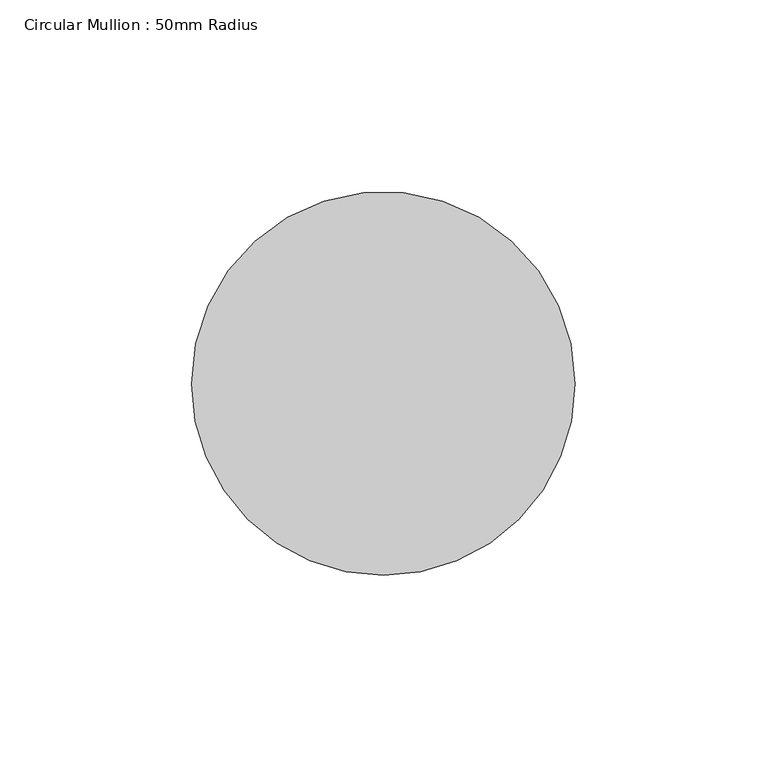
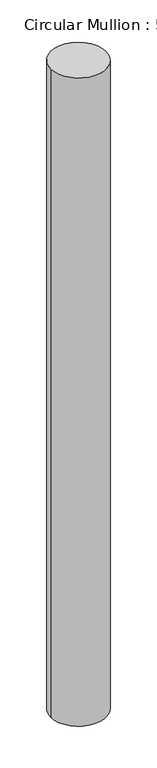
"""IFC4 building model written with IfcOpenShell, lengths in millimetres: member geometry, Circular Mullion : 50mm Radius."""

from ifc_helpers import new_model, si_unit, frame, origin, place, context, project, spatial, ellipse_curve, source, transform, mapped, element, save
from ifc_brep_helpers import plane_surface, cylinder_surface, advanced_brep


def circular_mullion_50mm_radius_11ac74c6(model_context):
    return source(origin(), model_context, "Body", "AdvancedBrep", [
        advanced_brep(
        [(-100.0, 0.0, 0.6910365), (0.0, 0.0, 0.0), (0.0, 0.0, -1242.7098451), (-100.0, 0.0, -1243.4311044)],
        [
            (0, 1, ellipse_curve(frame((-50.0, 0.0, 0.3455183), z_axis=(-0.006909628578011499, -0.012865343381346107, -0.999893364300711), x_axis=(-0.47310077416802043, -0.88088727851764, 0.014603425194297921)), 50.0053324, 50.0)),
            (1, 2),
            (2, 3, ellipse_curve(frame((-50.0, 0.0, -1243.0704748), z_axis=(-0.007211755555192615, -0.013427886977189473, 0.9998838344693548), x_axis=(0.4730962651165488, 0.8808788829151897, 0.015241967289685193)), 50.005809, 50.0)),
            (3, 0),
            (1, 0, ellipse_curve(frame((-50.0, 0.0, 0.3455183), z_axis=(-0.006909628578011499, -0.012865343381346107, -0.999893364300711), x_axis=(-0.47310077416802043, -0.88088727851764, 0.014603425194297921)), 50.0053324, 50.0)),
            (3, 2, ellipse_curve(frame((-50.0, 0.0, -1243.0704748), z_axis=(-0.007211755555192615, -0.013427886977189473, 0.9998838344693548), x_axis=(0.4730962651165488, 0.8808788829151897, 0.015241967289685193)), 50.005809, 50.0)),
        ],
        [
            cylinder_surface(frame((-50.0, 0.0, 0.0), z_axis=(0.0, 0.0, 1.0), x_axis=(1.0, 0.0, 0.0)), 50.0),
            plane_surface(frame((-268.5230766, 144.2164946, 0.0), z_axis=(0.006909628578011499, 0.012865343381346107, 0.999893364300711), x_axis=(0.47310077416801877, 0.8808872785176406, -0.01460342519431723))),
            plane_surface(frame((-268.5230766, 144.2164946, -1242.7098451), z_axis=(0.007211755555192615, 0.013427886977189473, -0.9998838344693548), x_axis=(0.47309626511654873, 0.8808788829151896, 0.015241967289691516))),
        ],
        [
            (0, [[1, 2, 3, 4]]),
            (0, [[5, -4, 6, -2]]),
            (1, [[-1, -5]]),
            (2, [[-6, -3]]),
        ],
    ),
    ])


if __name__ == "__main__":
    model = new_model("IFC4")
    model_context = context("Model", 3, world=origin())
    ifc_project = project(units=[si_unit("LENGTHUNIT", "METRE", prefix="MILLI")], contexts=[model_context])
    site = spatial("IfcSite", under=ifc_project)
    building = spatial("IfcBuilding", under=site)
    placement = place(None, origin())
    circular_mullion_50mm_radius_shape = circular_mullion_50mm_radius_11ac74c6(model_context)
    element("IfcMember", 1, ObjectType="Circular Mullion : 50mm Radius", at=placement, inside=building, context=model_context, shape_type="MappedRepresentation", body=[
        mapped(circular_mullion_50mm_radius_shape, transform((0.0, 0.0, 0.0), x_axis=(1.0, 0.0, 0.0), y_axis=(0.0, 1.0, 0.0), z_axis=(0.0, 0.0, 1.0))),
    ])
    save(model, "model.ifc")

# Revit data of these elements
# Type "Circular Mullion : 50mm Radius"
#   built-in parameter 1007350 = 0.164042 (stored number, unit not read)
# Element 1 (IfcMember, "Circular Mullion : 50mm Radius")
#   Materials on its faces: "Aluminium"
# Materials
#   "Aluminium": class "Metal", colour RGB 247 247 247, transparency 0, Description = "Aluminium 6061", Cost = 0
